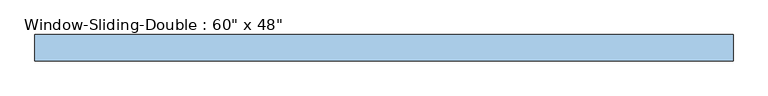
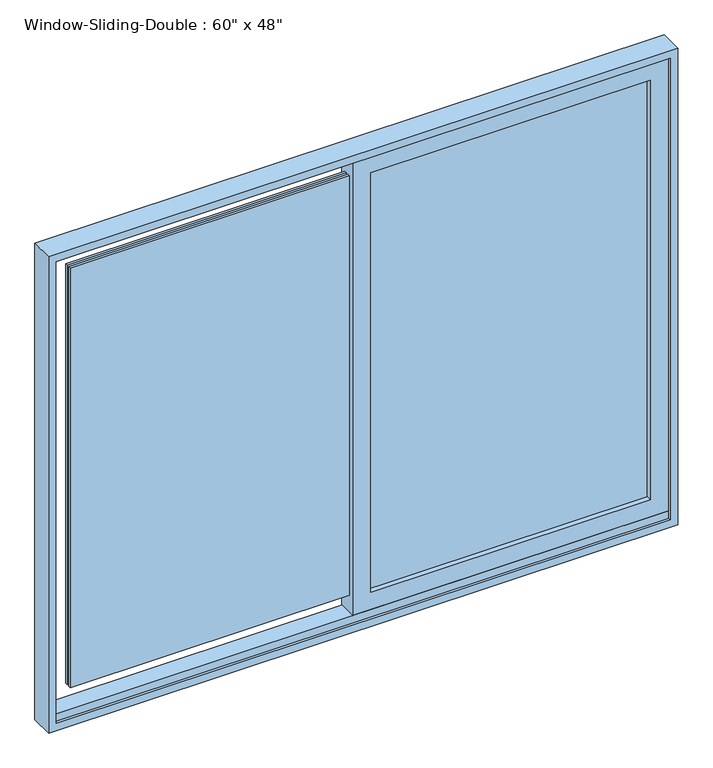
"""IFC4 building model written with IfcOpenShell, lengths in millimetres: window geometry."""

from ifc_helpers import new_model, si_unit, frame, origin, place, context, project, spatial, polyline, outline, extrude, faceted_brep, source, transform, mapped, element, save


def window_be6137b3(model_context):
    return source(origin(), model_context, "Body", "SolidModel", [
        faceted_brep([(-762.0, -10.16, 914.4), (-762.0, 46.99, 914.4), (762.0, 46.99, 914.4), (762.0, -10.16, 914.4), (-721.0778905, 46.99, 2092.6778905), (-721.0778905, 40.64, 2092.6778905), (-721.0778905, 40.64, 952.5), (-721.0778905, 40.64, 933.45), (-721.0778905, 46.99, 933.45), (721.0778905, 40.64, 2092.6778905), (721.0778905, 40.64, 952.5), (742.95, 40.64, 952.5), (742.95, 40.64, 2114.55), (-742.95, 40.64, 2114.55), (-742.95, 40.64, 952.5), (-742.95, -10.16, 2114.55), (-742.95, -10.16, 933.45), (-742.95, -3.81, 933.45), (-742.95, -3.81, 952.5), (762.0, -10.16, 2133.6), (-762.0, -10.16, 2133.6), (742.95, -10.16, 2114.55), (742.95, -10.16, 933.45), (-762.0, 46.99, 2133.6), (762.0, 46.99, 2133.6), (721.0778905, 46.99, 933.45), (721.0778905, 46.99, 2092.6778905), (721.0778905, 40.64, 933.45), (742.95, -3.81, 952.5), (742.95, -3.81, 933.45)], [[[0, 1, 2, 3]], [[4, 5, 6, 7, 8]], [[5, 9, 10, 11, 12, 13, 14, 6]], [[13, 15, 16, 17, 18, 14]], [[0, 3, 19, 20], [21, 22, 16, 15]], [[23, 1, 0, 20]], [[2, 1, 23, 24], [4, 8, 25, 26]], [[5, 4, 26, 9]], [[13, 12, 21, 15]], [[20, 19, 24, 23]], [[9, 26, 25, 27, 10]], [[21, 12, 11, 28, 29, 22]], [[19, 3, 2, 24]], [[7, 27, 25, 8]], [[27, 7, 6, 10]], [[10, 6, 14, 18, 28, 11]], [[28, 18, 17, 29]], [[16, 22, 29, 17]]]),
        extrude(outline(polyline([(698.5, 27.94), (698.5, 21.59), (22.225, 21.59), (22.225, 27.94), (698.5, 27.94)])), frame((0.0, 0.0, 996.95), z_axis=(0.0, 0.0, 1.0), x_axis=(1.0, 0.0, 0.0)), (0.0, 0.0, 1.0), 1073.15),
        extrude(outline(polyline([(698.5, 15.24), (698.5, 8.89), (22.225, 8.89), (22.225, 15.24), (698.5, 15.24)])), frame((0.0, 0.0, 996.95), z_axis=(0.0, 0.0, 1.0), x_axis=(1.0, 0.0, 0.0)), (0.0, 0.0, 1.0), 1073.15),
        extrude(outline(polyline([(-22.225, 27.94), (-22.225, 21.59), (-698.5, 21.59), (-698.5, 27.94), (-22.225, 27.94)])), frame((0.0, 0.0, 996.95), z_axis=(0.0, 0.0, 1.0), x_axis=(1.0, 0.0, 0.0)), (0.0, 0.0, 1.0), 1073.15),
        extrude(outline(polyline([(-22.225, 15.24), (-22.225, 8.89), (-698.5, 8.89), (-698.5, 15.24), (-22.225, 15.24)])), frame((0.0, 0.0, 996.95), z_axis=(0.0, 0.0, 1.0), x_axis=(1.0, 0.0, 0.0)), (0.0, 0.0, 1.0), 1073.15),
        extrude(outline(polyline([(952.5, 742.95), (2114.55, 742.95), (2114.55, -22.225), (952.5, -22.225), (952.5, 742.95)]), holes=[polyline([(996.95, 22.225), (2070.1, 22.225), (2070.1, 698.5), (996.95, 698.5), (996.95, 22.225)])]), frame((0.0, -3.81, 0.0), z_axis=(0.0, 1.0, 0.0), x_axis=(0.0, 0.0, 1.0)), (0.0, 0.0, 1.0), 44.45),
    ])


if __name__ == "__main__":
    model = new_model("IFC4")
    model_context = context("Model", 3, world=origin())
    ifc_project = project(units=[si_unit("LENGTHUNIT", "METRE", prefix="MILLI")], contexts=[model_context])
    site = spatial("IfcSite", under=ifc_project)
    building = spatial("IfcBuilding", under=site)
    placement = place(None, origin())
    window_shape = window_be6137b3(model_context)
    element("IfcWindow", 1, ObjectType="Window-Sliding-Double : 60\" x 48\"", at=placement, inside=building, context=model_context, shape_type="MappedRepresentation", body=[
        mapped(window_shape, transform((0.0, 0.0, 0.0), x_axis=(1.0, 0.0, 0.0), y_axis=(0.0, 1.0, 0.0), z_axis=(0.0, 0.0, 1.0))),
    ])
    save(model, "model.ifc")

# Revit data of these elements
# Type "Window-Sliding-Double : 60\" x 48\""
#   Type Mark = "22"
#   Fire Rating = "0.5h"
#   Assembly Code = "B2020100"
#   Analytic Construction = "Double glazing - domestic"
#   Window Inset [instance default] = 0' - 0"
#   Wall Thickness [instance default] = 0' - 6"
#   Visual Light Transmittance = 0.81
#   Thermal Resistance (R) = 1.8146 (h·ft²·°F)/BTU
#   Solar Heat Gain Coefficient = 0.76
#   Muntin Width = 2' - 2 5/8"
#   Muntin Height = 3' - 6 1/4"
#   Interior Wall Closure [instance default] = 0' - 2 3/4"
#   Heat Transfer Coefficient (U) = 0.5511 BTU/(h·ft²·°F)
#   Frame Extension [instance default] = 0' - 0 1/4"
#   Exterior Wall Closure [instance default] = 0' - 1 1/4"
#   Rough Width = 5' - 0 1/2"
#   Rough Height = 4' - 0 1/2"
#   Height = 4' - 0"
#   Extension Jamb [instance default] = 0' - 2 3/4"
#   Default Sill Height = 3' - 0"
#   Width = 5' - 0"
#   Interior Trim Visibility [instance default] = yes
#   Indicator Visibility [instance default] = yes
#   Exterior Trim Visibility [instance default] = yes
#   Muntin Visibility = yes
#   Extension Jamb Visibility [instance default] = yes
#   Muntin Pattern = Muntin Pattern_2x2 : Muntin Pattern_2x2
#   Interior Trim Material = Wood - Stained
#   Interior Trim = Trim-Window-Interior-Flat : Picture Frame
#   Interior Frame Material = Wood - Stained
#   Glass Panel Material = Glass
#   Exterior Trim Material = Clad - White
#   Exterior Trim = Trim-Window-Exterior-Flat : with Sill
#   Exterior Frame Material = Clad - White
#   Wall Closure = (empty or 0)
# Element 1 (IfcWindow, "Window-Sliding-Double : 60\" x 48\"")
#   Wall Thickness = 0' - 2 1/2"
#   Extension Jamb = 0' - 1"
#   Extension Jamb Visibility = no
#   Materials on its faces: "Glass", "Wood - Stained", "Clad - White"
# Materials
#   "Wood - Stained": class "Wood", colour RGB 224 178 126, transparency 0, Cost = 0
#   "Glass": class "Glass", colour RGB 0 128 192, transparency 0.75, Description = "Soda Lime Glass", Cost = 0
#   "Clad - White": class "Wood", colour RGB 242 242 238, transparency 0, Cost = 0
